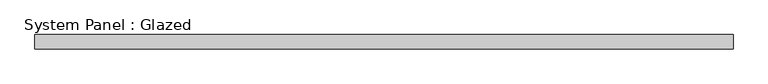
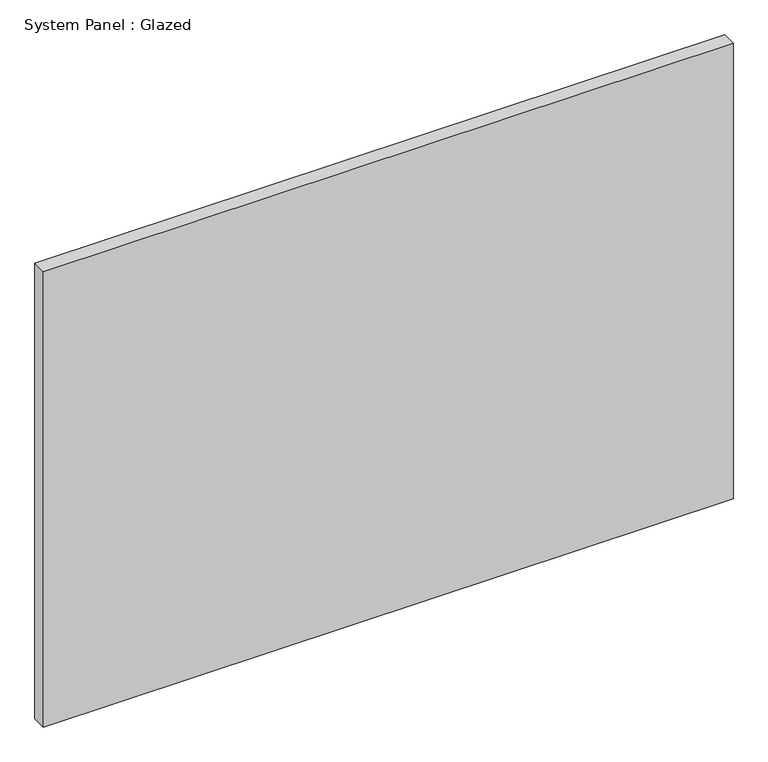
"""IFC4 building model written with IfcOpenShell, lengths in millimetres: plate geometry, System Panel : Glazed."""

import ifcopenshell
import ifcopenshell.guid

model = None  # the IFC model being written
_history = None  # IfcOwnerHistory: only IFC2X3 demands one
_inside = {}  # id of a spatial element -> (the spatial element, [elements in it])
_under = {}  # id of a project, library or spatial element -> (it, [spatial elements below it])
_declared = {}  # id of a project -> (the project, [libraries it declares])
_typed = {}  # id of a type object -> (the type object, [elements of that type])
_made_of = {}  # id of a material, layer set ... -> (it, [elements and type objects made of it])


def new_model(schema):
    """Start an empty IFC model of exactly this schema.

    Asked for "IFC4X3", IfcOpenShell would pick the latest addendum, in which some entities
    have other attributes; the version numbers below select the first issue.
    IFC2X3 requires an IfcOwnerHistory on every rooted entity: one is made here for all.
    """
    global model, _history
    if schema == "IFC4X3":
        model = ifcopenshell.file(schema_version=(4, 3, 0, 0))
    else:
        model = ifcopenshell.file(schema=schema)
    _inside.clear()
    _under.clear()
    _declared.clear()
    _typed.clear()
    _made_of.clear()
    _history = None
    if model.schema == "IFC2X3":
        org = make("IfcOrganization", Name="unknown")
        user = make(
            "IfcPersonAndOrganization",
            ThePerson=make("IfcPerson", FamilyName="unknown"),
            TheOrganization=org,
        )
        app = make(
            "IfcApplication",
            ApplicationDeveloper=org,
            Version="unknown",
            ApplicationFullName="unknown",
            ApplicationIdentifier="unknown",
        )
        _history = make(
            "IfcOwnerHistory",
            OwningUser=user,
            OwningApplication=app,
            ChangeAction="ADDED",
            CreationDate=0,
        )
    return model


def make(cls, **values):
    """One entity of the class cls with the attributes given. An attribute that is None is left unset."""
    return model.create_entity(
        cls, **{name: value for name, value in values.items() if value is not None}
    )


def rooted(cls, **values):
    """An entity with a GlobalId (a new one), such as an element, a storey or a relation."""
    return make(cls, GlobalId=ifcopenshell.guid.new(), OwnerHistory=_history, **values)


def si_unit(unit_type, name, prefix=None):
    """IfcSIUnit, for example si_unit("LENGTHUNIT", "METRE", prefix="MILLI")."""
    return make("IfcSIUnit", UnitType=unit_type, Prefix=prefix, Name=name)


def assignment(units):
    """IfcUnitAssignment: the units of a project."""
    return None if units is None else make("IfcUnitAssignment", Units=units)


def point(xyz):
    """IfcCartesianPoint."""
    return None if xyz is None else make("IfcCartesianPoint", Coordinates=xyz)


def direction(xyz):
    """IfcDirection."""
    return None if xyz is None else make("IfcDirection", DirectionRatios=xyz)


def frame(location, z_axis=None, x_axis=None):
    """IfcAxis2Placement3D, a coordinate frame: its origin and axes. An axis left out is left unset."""
    return make(
        "IfcAxis2Placement3D",
        Location=point(location),
        Axis=direction(z_axis),
        RefDirection=direction(x_axis),
    )


def origin():
    """The frame at (0, 0, 0) with its axes left unset."""
    return frame((0.0, 0.0, 0.0))


def origin_with_axes():
    """The frame at (0, 0, 0) with the z axis (0, 0, 1) and the x axis (1, 0, 0) written out."""
    return frame((0.0, 0.0, 0.0), z_axis=(0.0, 0.0, 1.0), x_axis=(1.0, 0.0, 0.0))


def place(relative_to, where):
    """IfcLocalPlacement: puts the frame where relative to a parent placement (None: the world)."""
    return make(
        "IfcLocalPlacement", PlacementRelTo=relative_to, RelativePlacement=where
    )


def context(
    kind, dimensions, precision=None, world=None, true_north=None, identifier=None
):
    """IfcGeometricRepresentationContext, for example the 3D "Model" context."""
    return make(
        "IfcGeometricRepresentationContext",
        ContextIdentifier=identifier,
        ContextType=kind,
        CoordinateSpaceDimension=dimensions,
        Precision=precision,
        WorldCoordinateSystem=world,
        TrueNorth=true_north,
    )


def project(units=None, contexts=None):
    """IfcProject with its units and contexts."""
    return rooted(
        "IfcProject",
        Name="project",
        RepresentationContexts=contexts,
        UnitsInContext=assignment(units),
    )


def spatial(cls, under=None, at=None, **own):
    """A site, building, storey or space (cls), placed at a placement, below another one or the project."""
    s = rooted(cls, ObjectPlacement=at, **own)
    if under is not None:
        _under.setdefault(under.id(), (under, []))[1].append(s)
    return s


def polyline(points):
    """IfcPolyline through the points."""
    return make("IfcPolyline", Points=[point(p) for p in points])


def outline(outer, holes=None, kind="AREA"):
    """IfcArbitraryClosedProfileDef: a profile drawn as a closed curve; with holes, ...WithVoids."""
    if holes is None:
        return make("IfcArbitraryClosedProfileDef", ProfileType=kind, OuterCurve=outer)
    return make(
        "IfcArbitraryProfileDefWithVoids",
        ProfileType=kind,
        OuterCurve=outer,
        InnerCurves=holes,
    )


def extrude(swept, where, along, depth):
    """IfcExtrudedAreaSolid: the profile swept, set in the frame where, extruded along a direction by depth."""
    return make(
        "IfcExtrudedAreaSolid",
        SweptArea=swept,
        Position=where,
        ExtrudedDirection=direction(along),
        Depth=depth,
    )


def shape(context_of_items, identifier, shape_type, items):
    """IfcShapeRepresentation: the items that make up one representation, for example the "Body"."""
    return make(
        "IfcShapeRepresentation",
        ContextOfItems=context_of_items,
        RepresentationIdentifier=identifier,
        RepresentationType=shape_type,
        Items=items,
    )


def source(mapping_origin, context_of_items, identifier, shape_type, items):
    """IfcRepresentationMap: a shape defined once, which mapped items show again and again."""
    return make(
        "IfcRepresentationMap",
        MappingOrigin=mapping_origin,
        MappedRepresentation=shape(context_of_items, identifier, shape_type, items),
    )


def transform(
    local_origin,
    x_axis=None,
    y_axis=None,
    z_axis=None,
    scale=None,
    scale2=None,
    scale3=None,
    uniform=True,
):
    """IfcCartesianTransformationOperator3D, or its non-uniform kind. x_axis, y_axis, z_axis: its Axis1, 2, 3."""
    if uniform:
        return make(
            "IfcCartesianTransformationOperator3D",
            Axis1=direction(x_axis),
            Axis2=direction(y_axis),
            LocalOrigin=point(local_origin),
            Scale=scale,
            Axis3=direction(z_axis),
        )
    return make(
        "IfcCartesianTransformationOperator3DnonUniform",
        Axis1=direction(x_axis),
        Axis2=direction(y_axis),
        LocalOrigin=point(local_origin),
        Scale=scale,
        Axis3=direction(z_axis),
        Scale2=scale2,
        Scale3=scale3,
    )


def mapped(mapping_source, mapping_target):
    """IfcMappedItem: shows the shape of a source again, moved by a transform."""
    return make(
        "IfcMappedItem", MappingSource=mapping_source, MappingTarget=mapping_target
    )


def made_of(thing, what):
    """Note that an element or type object is made of a material, layer set ...; save() writes the relation."""
    if what is not None:
        _made_of.setdefault(what.id(), (what, []))[1].append(thing)
    return thing


def element(
    cls,
    number,
    at=None,
    inside=None,
    cuts=None,
    type_object=None,
    material=None,
    context=None,
    identifier="Body",
    shape_type=None,
    held_by="IfcProductDefinitionShape",
    body=None,
    shapes=None,
    **own,
):
    """One element of the class cls, such as IfcWall. Its Tag is "e" and its number.

    at: its placement. inside: the storey or other place that contains it. cuts: it is an
    opening in that element (IfcRelVoidsElement). A single representation is given by context,
    identifier, shape_type and body (its items); several are given by shapes. held_by: the class
    of the entity that holds the representations. save() writes the other relations.
    """
    e = rooted(cls, Tag="e%d" % number, ObjectPlacement=at, **own)
    if body is not None:
        shapes = [shape(context, identifier, shape_type, body)]
    if shapes is not None:
        e.Representation = make(held_by, Representations=shapes)
    if inside is not None:
        _inside.setdefault(inside.id(), (inside, []))[1].append(e)
    if cuts is not None:
        rooted(
            "IfcRelVoidsElement", RelatingBuildingElement=cuts, RelatedOpeningElement=e
        )
    if type_object is not None:
        _typed.setdefault(type_object.id(), (type_object, []))[1].append(e)
    return made_of(e, material)


def aggregate(whole, parts):
    """IfcRelAggregates: a whole, such as a stair, and the parts it consists of."""
    return rooted("IfcRelAggregates", RelatingObject=whole, RelatedObjects=parts)


def save(model, path):
    """Write the relations noted so far, then the file.

    IfcRelAggregates (storeys below a building ...), IfcRelContainedInSpatialStructure (elements
    in a storey), IfcRelDefinesByType, IfcRelAssociatesMaterial and IfcRelDeclares: one each for
    every whole, place, type object, material and project.
    """
    for whole, parts in _under.values():
        aggregate(whole, parts)
    for where, things in _inside.values():
        rooted(
            "IfcRelContainedInSpatialStructure",
            RelatedElements=things,
            RelatingStructure=where,
        )
    for kind, things in _typed.values():
        rooted("IfcRelDefinesByType", RelatedObjects=things, RelatingType=kind)
    for what, things in _made_of.values():
        rooted("IfcRelAssociatesMaterial", RelatedObjects=things, RelatingMaterial=what)
    for by, libraries in _declared.values():
        rooted("IfcRelDeclares", RelatingContext=by, RelatedDefinitions=libraries)
    model.write(path)


def system_panel_glazed_8fe7ab7d(model_context):
    return source(origin(), model_context, "Body", "SweptSolid", [
        extrude(outline(polyline([(609.6, 19.05), (-609.6, 19.05), (-609.6, 44.45), (609.6, 44.45), (609.6, 19.05)])), origin_with_axes(), (0.0, 0.0, 1.0), 850.9),
    ])


if __name__ == "__main__":
    model = new_model("IFC4")
    model_context = context("Model", 3, world=origin())
    ifc_project = project(units=[si_unit("LENGTHUNIT", "METRE", prefix="MILLI")], contexts=[model_context])
    site = spatial("IfcSite", under=ifc_project)
    building = spatial("IfcBuilding", under=site)
    placement = place(None, origin())
    system_panel_glazed_shape = system_panel_glazed_8fe7ab7d(model_context)
    element("IfcPlate", 1, ObjectType="System Panel : Glazed", at=placement, inside=building, context=model_context, shape_type="MappedRepresentation", body=[
        mapped(system_panel_glazed_shape, transform((0.0, 0.0, 0.0), x_axis=(1.0, 0.0, 0.0), y_axis=(0.0, 1.0, 0.0), z_axis=(0.0, 0.0, 1.0))),
    ])
    save(model, "model.ifc")

# Revit data of these elements
# Type "System Panel : Glazed"
#   Construction Type Id = "GSP4R"
#   Analytic Construction = "1/8 in Pilkington single glazing"
#   Visual Light Transmittance = 0.9
#   Solar Heat Gain Coefficient = 0.86
#   Heat Transfer Coefficient (U) = 1.18115 BTU/(h·ft²·°F)
#   Define Thermal Properties by = 1
# Element 1 (IfcPlate, "System Panel : Glazed")
#   Materials on its faces: "Glass"
# Materials
#   "Glass": class "Glass", colour RGB 0 128 192, transparency 0.75, Description = "Soda Lime Glass", Cost = 0
